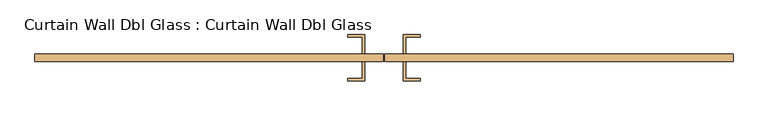
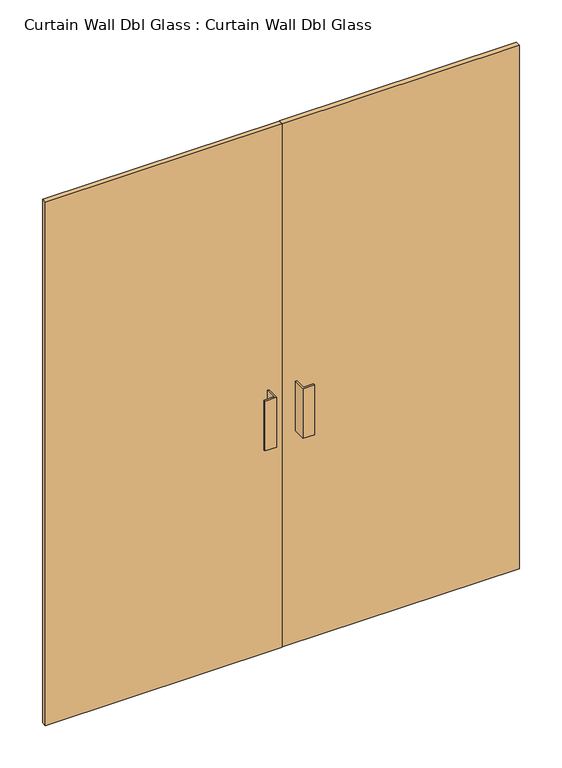
"""IFC4 building model written with IfcOpenShell, lengths in millimetres: door geometry, Curtain Wall Dbl Glass : Curtain Wall Dbl Glass."""

from ifc_helpers import new_model, si_unit, frame, origin, origin_with_axes, place, context, project, spatial, polyline, outline, extrude, source, transform, mapped, element, save


def curtain_wall_dbl_glass_curtain_wall_dbl_glass_a5de0235(model_context):
    return source(origin(), model_context, "Body", "SweptSolid", [
        extrude(outline(polyline([(-1.5875, -31.75), (-1.5875, -50.8), (-914.4, -50.8), (-914.4, -31.75), (-1.5875, -31.75)])), origin_with_axes(), (0.0, 0.0, 1.0), 2133.6),
        extrude(outline(polyline([(914.4, -31.75), (914.4, -50.8), (1.5875, -50.8), (1.5875, -31.75), (914.4, -31.75)])), origin_with_axes(), (0.0, 0.0, 1.0), 2133.6),
        extrude(outline(polyline([(-50.8, -101.6), (-95.25, -101.6), (-95.25, -95.25), (-57.15, -95.25), (-57.15, -50.8), (-50.8, -50.8), (-50.8, -101.6)])), frame((0.0, 0.0, 863.6), z_axis=(0.0, 0.0, 1.0), x_axis=(1.0, 0.0, 0.0)), (0.0, 0.0, 1.0), 203.2),
        extrude(outline(polyline([(50.8, -101.6), (50.8, -50.8), (57.15, -50.8), (57.15, -95.25), (95.25, -95.25), (95.25, -101.6), (50.8, -101.6)])), frame((0.0, 0.0, 863.6), z_axis=(0.0, 0.0, 1.0), x_axis=(1.0, 0.0, 0.0)), (0.0, 0.0, 1.0), 203.2),
        extrude(outline(polyline([(-50.8, 19.05), (-50.8, -31.75), (-57.15, -31.75), (-57.15, 12.7), (-95.25, 12.7), (-95.25, 19.05), (-50.8, 19.05)])), frame((0.0, 0.0, 863.6), z_axis=(0.0, 0.0, 1.0), x_axis=(1.0, 0.0, 0.0)), (0.0, 0.0, 1.0), 203.2),
        extrude(outline(polyline([(50.8, 19.05), (95.25, 19.05), (95.25, 12.7), (57.15, 12.7), (57.15, -31.75), (50.8, -31.75), (50.8, 19.05)])), frame((0.0, 0.0, 863.6), z_axis=(0.0, 0.0, 1.0), x_axis=(1.0, 0.0, 0.0)), (0.0, 0.0, 1.0), 203.2),
    ])


if __name__ == "__main__":
    model = new_model("IFC4")
    model_context = context("Model", 3, world=origin())
    ifc_project = project(units=[si_unit("LENGTHUNIT", "METRE", prefix="MILLI")], contexts=[model_context])
    site = spatial("IfcSite", under=ifc_project)
    building = spatial("IfcBuilding", under=site)
    placement = place(None, origin())
    curtain_wall_dbl_glass_curtain_wall_dbl_glass_shape = curtain_wall_dbl_glass_curtain_wall_dbl_glass_a5de0235(model_context)
    element("IfcDoor", 1, ObjectType="Curtain Wall Dbl Glass : Curtain Wall Dbl Glass", at=placement, inside=building, context=model_context, shape_type="MappedRepresentation", body=[
        mapped(curtain_wall_dbl_glass_curtain_wall_dbl_glass_shape, transform((0.0, 0.0, 0.0), x_axis=(1.0, 0.0, 0.0), y_axis=(0.0, 1.0, 0.0), z_axis=(0.0, 0.0, 1.0))),
    ])
    save(model, "model.ifc")

# Revit data of these elements
# Type "Curtain Wall Dbl Glass : Curtain Wall Dbl Glass"
#   Offset = 0' - 2"
#   Function = 1
#   Handle Material = Metal - Aluminum
#   Glazing Material = Glass
# Element 1 (IfcDoor, "Curtain Wall Dbl Glass : Curtain Wall Dbl Glass")
#   Materials on its faces: "Metal - Aluminum", "Glass"
# Materials
#   "Metal - Aluminum": class "Metal", colour RGB 140 140 140, transparency 0
#   "Glass": class "Glass", colour RGB 0 128 192, transparency 0.75
